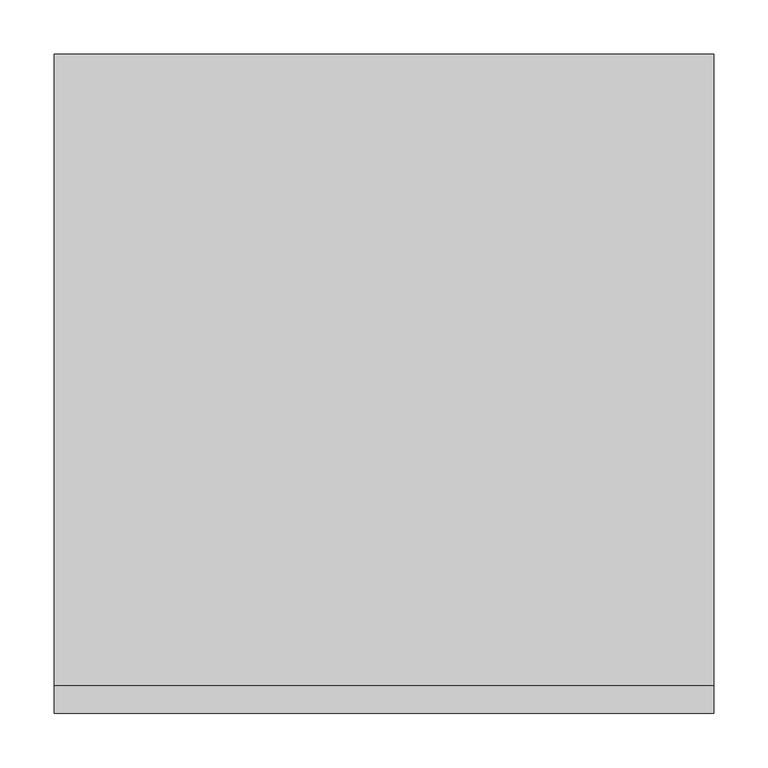
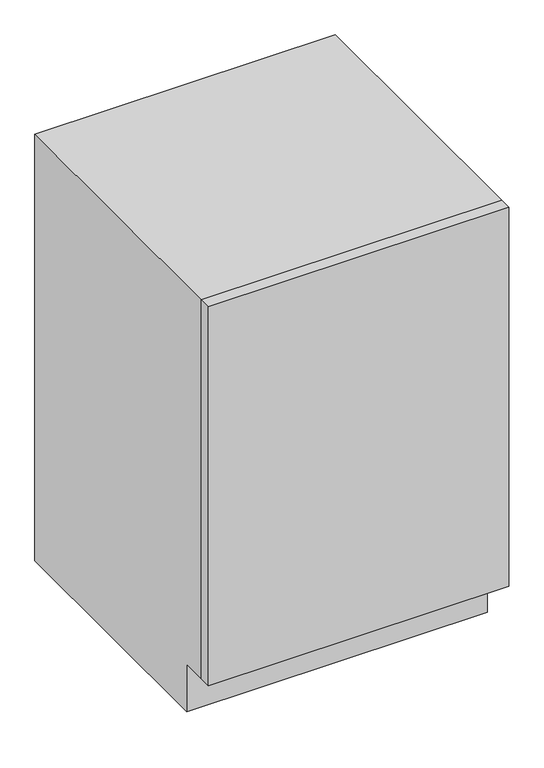
"""IFC4 building model written with IfcOpenShell, lengths in millimetres: furniture geometry, OD_CW_Base Cabinet : OD_CW_Base Cabinet."""

from ifc_helpers import new_model, si_unit, frame, origin, place, context, project, spatial, polyline, outline, extrude, source, transform, mapped, element, save


def furniture_55236fef(model_context):
    return source(origin(), model_context, "Body", "SweptSolid", [
        extrude(outline(polyline([(18.7377049, 25.4), (628.3377049, 25.4), (628.3377049, 0.0), (18.7377049, 0.0), (18.7377049, 25.4)])), frame((0.0, 0.0, 101.6), z_axis=(0.0, 0.0, 1.0), x_axis=(1.0, 0.0, 0.0)), (0.0, 0.0, 1.0), 812.8),
        extrude(outline(polyline([(25.4, 914.4), (609.6, 914.4), (609.6, 0.0), (76.2, 0.0), (76.2, 101.6), (25.4, 101.6), (25.4, 914.4)])), frame((18.7377049, 0.0, 0.0), z_axis=(1.0, 0.0, 0.0), x_axis=(0.0, 1.0, 0.0)), (0.0, 0.0, 1.0), 609.6),
    ])


if __name__ == "__main__":
    model = new_model("IFC4")
    model_context = context("Model", 3, world=origin())
    ifc_project = project(units=[si_unit("LENGTHUNIT", "METRE", prefix="MILLI")], contexts=[model_context])
    site = spatial("IfcSite", under=ifc_project)
    building = spatial("IfcBuilding", under=site)
    placement = place(None, origin())
    furniture_shape = furniture_55236fef(model_context)
    element("IfcFurniture", 1, ObjectType="OD_CW_Base Cabinet : OD_CW_Base Cabinet", at=placement, inside=building, context=model_context, shape_type="MappedRepresentation", body=[
        mapped(furniture_shape, transform((0.0, 0.0, 0.0), x_axis=(1.0, 0.0, 0.0), y_axis=(0.0, 1.0, 0.0), z_axis=(0.0, 0.0, 1.0))),
    ])
    save(model, "model.ifc")

# Revit data of these elements
# Type "OD_CW_Base Cabinet : OD_CW_Base Cabinet"
#   OD_CW_Width [instance default] = 2' - 10"
#   OD_CW_Length [instance default] = 8' - 0"
#   OD_CW_Height [instance default] = 2' - 3"
#   Depth = 2' - 0"
#   Height = 3' - 0"
#   Width = 4' - 0"
#   OD_CW_Material_Front Panel [instance default] = none
#   OD_CW_Material_Body [instance default] = none
# Element 1 (IfcFurniture, "OD_CW_Base Cabinet : OD_CW_Base Cabinet")
#   OD_CW_Width = 2' - 0"
#   OD_CW_Length = 2' - 0"
#   OD_CW_Height = 3' - 0"
#   OD_CW_Material_Body = WOOD SHELVES
#   Materials on its faces: "WOOD SHELVES", "CASEWORK"
# Materials
#   "WOOD SHELVES": class "Generic", colour RGB 187 187 187, transparency 0, Cost = 0
#   "CASEWORK": class "Generic", colour RGB 181 181 181, transparency 0, Cost = 0
